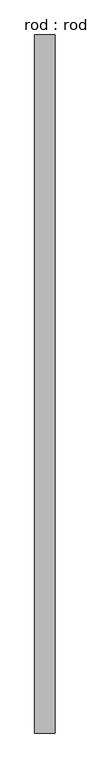
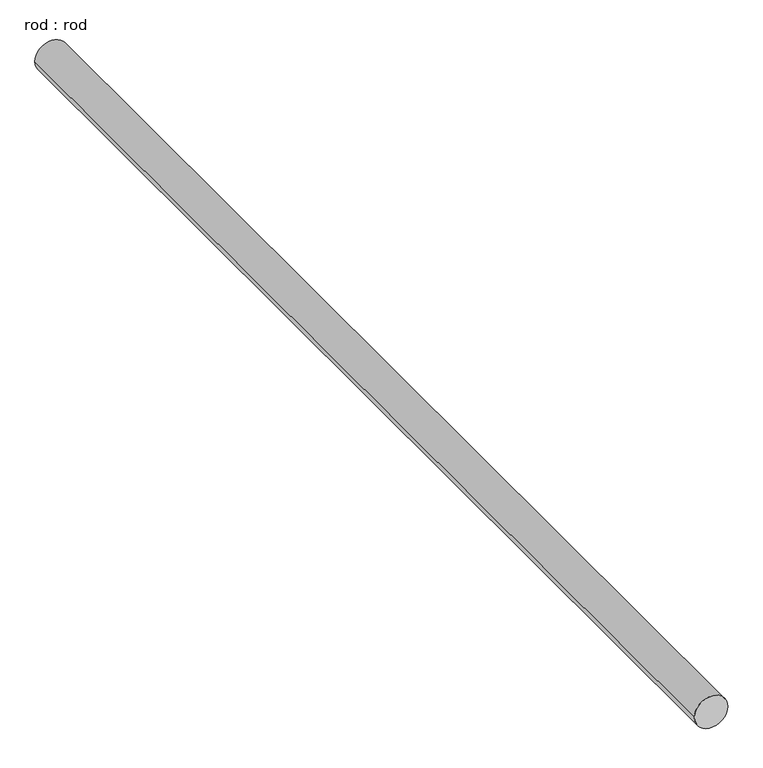
"""IFC4 building model written with IfcOpenShell, lengths in millimetres: proxy geometry, rod : rod."""

from ifc_helpers import new_model, si_unit, point, frame, frame_2d, origin, place, context, project, spatial, circle_curve, trimmed, segment, composite_curve, outline, extrude, source, transform, mapped, element, save


def rod_rod_826e77e5(model_context):
    return source(origin(), model_context, "Body", "SweptSolid", [
        extrude(outline(composite_curve([segment(trimmed(circle_curve(frame_2d((0.0108462, 0.0)), 200.0), [point((0.0108462, 200.0))], [point((0.0108462, -200.0))], False, "CARTESIAN"), True, "CONTINUOUS"), segment(trimmed(circle_curve(frame_2d((0.0108462, 0.0)), 200.0), [point((0.0108462, -200.0))], [point((0.0108462, 200.0))], False, "CARTESIAN"), True, "CONTINUOUS")], self_intersect=False)), frame((0.0, -2782.2845665, 0.0), z_axis=(0.0, 1.0, 0.0), x_axis=(0.0, 0.0, 1.0)), (0.0, 0.0, 1.0), 13750.0263636),
    ])


if __name__ == "__main__":
    model = new_model("IFC4")
    model_context = context("Model", 3, world=origin())
    ifc_project = project(units=[si_unit("LENGTHUNIT", "METRE", prefix="MILLI")], contexts=[model_context])
    site = spatial("IfcSite", under=ifc_project)
    building = spatial("IfcBuilding", under=site)
    placement = place(None, origin())
    rod_rod_shape = rod_rod_826e77e5(model_context)
    element("IfcBuildingElementProxy", 1, Name="rod : rod", ObjectType="rod : rod", at=placement, inside=building, context=model_context, shape_type="MappedRepresentation", body=[
        mapped(rod_rod_shape, transform((0.0, 0.0, 0.0), x_axis=(1.0, 0.0, 0.0), y_axis=(0.0, 1.0, 0.0), z_axis=(0.0, 0.0, 1.0))),
    ])
    save(model, "model.ifc")

# Revit data of these elements
# Type "rod : rod"
#   Default Elevation = 0
